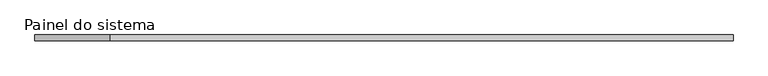
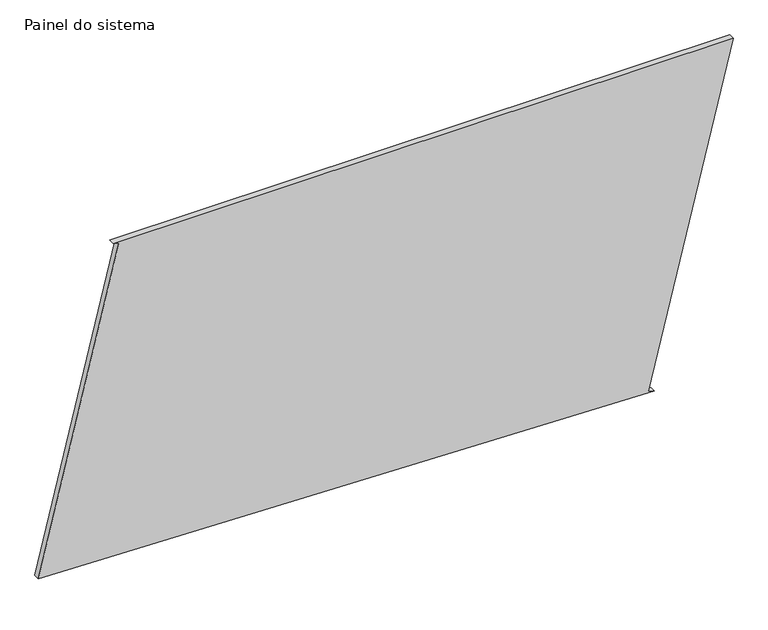
"""IFC4 building model written with IfcOpenShell, lengths in millimetres: plate geometry, Painel do sistema : Envidraçado."""

from ifc_helpers import new_model, si_unit, frame, origin, place, context, project, spatial, polyline, outline, extrude, source, transform, mapped, element, save


def painel_do_sistema_2862d4f7(model_context):
    return source(origin(), model_context, "Body", "SweptSolid", [
        extrude(outline(polyline([(0.0, 1135.8778197), (5.9765403, 1111.6027096), (1462.6198898, 1470.2287926), (1462.6198898, -1153.4760391), (1456.6433495, -1129.2009291), (71.4792665, -1470.2287926), (0.0, 1135.8778197)])), frame((0.0, 24.5, 0.0), z_axis=(0.0, 1.0, 0.0), x_axis=(0.0, 0.0, 1.0)), (0.0, 0.0, 1.0), 25.0),
    ])


if __name__ == "__main__":
    model = new_model("IFC4")
    model_context = context("Model", 3, world=origin())
    ifc_project = project(units=[si_unit("LENGTHUNIT", "METRE", prefix="MILLI")], contexts=[model_context])
    site = spatial("IfcSite", under=ifc_project)
    building = spatial("IfcBuilding", under=site)
    placement = place(None, origin())
    painel_do_sistema_shape = painel_do_sistema_2862d4f7(model_context)
    element("IfcPlate", 1, ObjectType="Painel do sistema : Envidraçado", at=placement, inside=building, context=model_context, shape_type="MappedRepresentation", body=[
        mapped(painel_do_sistema_shape, transform((0.0, 0.0, 0.0), x_axis=(1.0, 0.0, 0.0), y_axis=(0.0, 1.0, 0.0), z_axis=(0.0, 0.0, 1.0))),
    ])
    save(model, "model.ifc")

# Revit data of these elements
# Type "Painel do sistema : Envidraçado"
#   Construction Type Id = "GSP4R"
#   Analytic Construction = "Vidraça única Pilkington 1/8 pol"
#   Visual Light Transmittance = 0.9
#   Solar Heat Gain Coefficient = 0.86
#   Heat Transfer Coefficient (U) = 6.7069 W/(m²·K)
# Element 1 (IfcPlate, "Painel do sistema : Envidraçado")
#   Materials on its faces: "Vidro"
# Materials
#   "Vidro": class "Vidro", colour RGB 0 128 192, transparency 0.9, Description = "Vidro de sílica", Cost = 0
